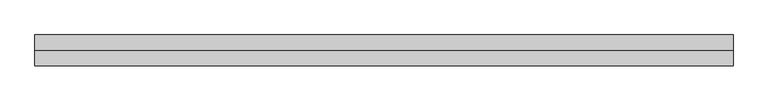
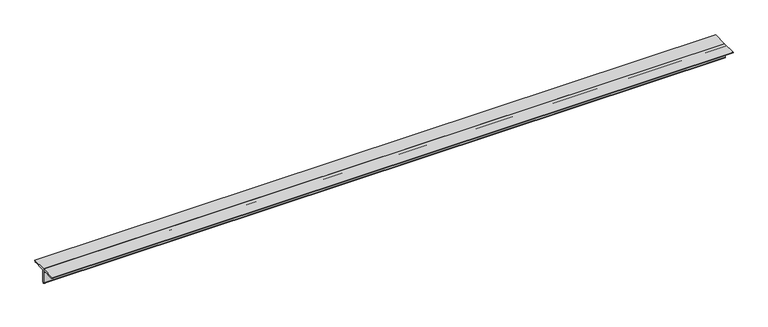
"""IFC4 building model written with IfcOpenShell, lengths in millimetres: member geometry, 0123_Steel Framing_2Ls-KSD3502 : H_SB_AR_S03_2Ls-130x130x12_HBR1."""

from ifc_helpers import new_model, si_unit, point, frame, frame_2d, origin, place, context, project, spatial, polyline, circle_curve, trimmed, segment, composite_curve, outline, extrude, source, transform, mapped, element, save


def member_5d0c7e09(model_context):
    return source(origin(), model_context, "Body", "SweptSolid", [
        extrude(outline(composite_curve([segment(polyline([(0.0, 36.4), (130.0, 36.4)]), True, "CONTINUOUS"), segment(trimmed(circle_curve(frame_2d((118.0, 36.4)), 12.0), [point((130.0, 36.4))], [point((118.0, 24.4))], False, "CARTESIAN"), True, "CONTINUOUS"), segment(polyline([(118.0, 24.4), (24.0, 24.4)]), True, "CONTINUOUS"), segment(trimmed(circle_curve(frame_2d((24.0, 12.4)), 12.0), [point((24.0, 24.4))], [point((12.0, 12.4))], True, "CARTESIAN"), True, "CONTINUOUS"), segment(polyline([(12.0, 12.4), (12.0, -81.6)]), True, "CONTINUOUS"), segment(trimmed(circle_curve(frame_2d((0.0, -81.6)), 12.0), [point((12.0, -81.6))], [point((0.0, -93.6))], False, "CARTESIAN"), True, "CONTINUOUS"), segment(polyline([(0.0, -93.6), (0.0, 36.4)]), True, "CONTINUOUS")], self_intersect=False)), frame((-2943.7629586, 0.0, 0.0), z_axis=(1.0, 0.0, 0.0), x_axis=(0.0, 1.0, 0.0)), (0.0, 0.0, 1.0), 5889.8945249),
        extrude(outline(composite_curve([segment(polyline([(0.0, 36.4), (0.0, -93.6)]), True, "CONTINUOUS"), segment(trimmed(circle_curve(frame_2d((0.0, -81.6)), 12.0), [point((0.0, -93.6))], [point((-12.0, -81.6))], False, "CARTESIAN"), True, "CONTINUOUS"), segment(polyline([(-12.0, -81.6), (-12.0, 12.4)]), True, "CONTINUOUS"), segment(trimmed(circle_curve(frame_2d((-24.0, 12.4)), 12.0), [point((-12.0, 12.4))], [point((-24.0, 24.4))], True, "CARTESIAN"), True, "CONTINUOUS"), segment(polyline([(-24.0, 24.4), (-118.0, 24.4)]), True, "CONTINUOUS"), segment(trimmed(circle_curve(frame_2d((-118.0, 36.4)), 12.0), [point((-118.0, 24.4))], [point((-130.0, 36.4))], False, "CARTESIAN"), True, "CONTINUOUS"), segment(polyline([(-130.0, 36.4), (0.0, 36.4)]), True, "CONTINUOUS")], self_intersect=False)), frame((-2943.7629586, 0.0, 0.0), z_axis=(1.0, 0.0, 0.0), x_axis=(0.0, 1.0, 0.0)), (0.0, 0.0, 1.0), 5889.8945249),
    ])


if __name__ == "__main__":
    model = new_model("IFC4")
    model_context = context("Model", 3, world=origin())
    ifc_project = project(units=[si_unit("LENGTHUNIT", "METRE", prefix="MILLI")], contexts=[model_context])
    site = spatial("IfcSite", under=ifc_project)
    building = spatial("IfcBuilding", under=site)
    placement = place(None, origin())
    member_shape = member_5d0c7e09(model_context)
    element("IfcMember", 1, ObjectType="0123_Steel Framing_2Ls-KSD3502 : H_SB_AR_S03_2Ls-130x130x12_HBR1", at=placement, inside=building, context=model_context, shape_type="MappedRepresentation", body=[
        mapped(member_shape, transform((0.0, 0.0, 0.0), x_axis=(1.0, 0.0, 0.0), y_axis=(0.0, 1.0, 0.0), z_axis=(0.0, 0.0, 1.0))),
    ])
    save(model, "model.ifc")

# Revit data of these elements
# Type "0123_Steel Framing_2Ls-KSD3502 : H_SB_AR_S03_2Ls-130x130x12_HBR1"
#   Assembly Code = "B10"
#   Legs = "SLBB"
#   W = 8.97
#   Perimeter = 1.04 m²/m
#   Nominal Weight = 46.80 kgf/m
#   Length [instance default] = 1000 mm
#   Space = 0 mm
#   b = 130 mm
#   d = 130 mm
#   t = 12 mm
#   y = 36.4 mm
#   A = 0.005952 m²
#   Structural Material [instance default] = Steel ASTM A36
# Element 1 (IfcMember, "0123_Steel Framing_2Ls-KSD3502 : H_SB_AR_S03_2Ls-130x130x12_HBR1")
#   Structural Material = Steel, 45-345
#   Materials on its faces: "Steel, 45-345"
# Materials
#   "Steel ASTM A36": class "Metal", colour RGB 199 199 199, transparency 0, Description = "Structural steel, ASTM A36 Grade B, mill finish", Cost = 0
#   "Steel, 45-345": class "Metal", colour RGB 189 187 185, transparency 0, Description = "Steel 345 MPa", Cost = 0
